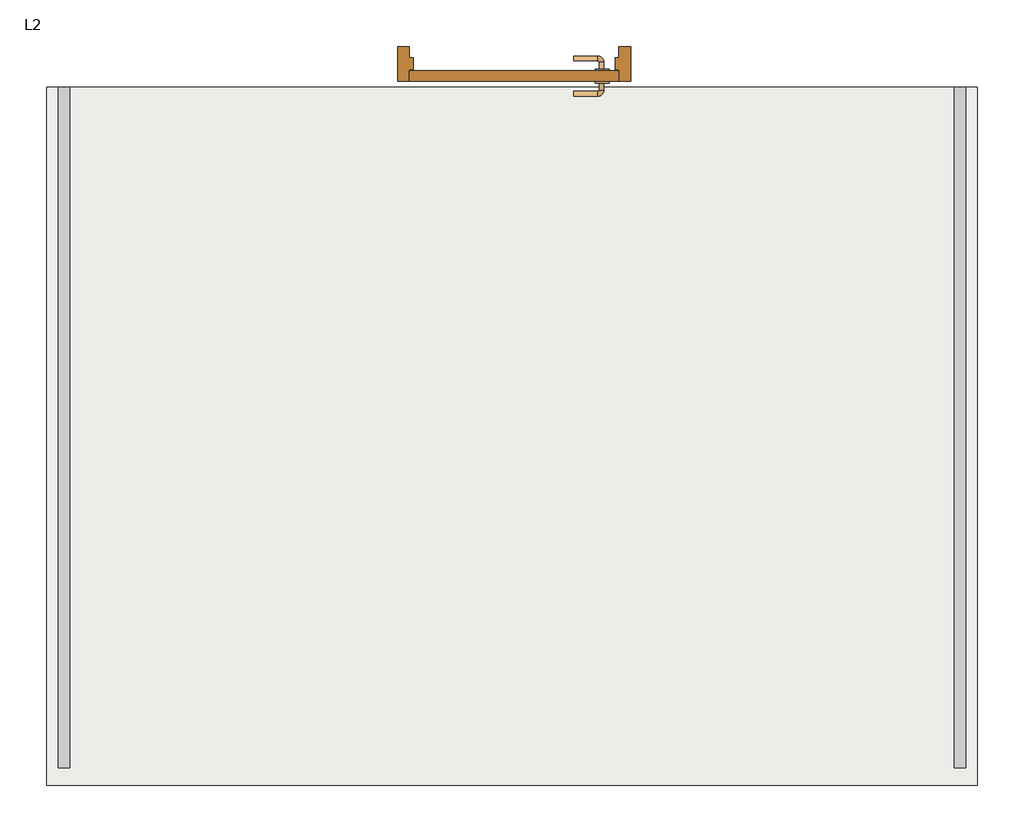
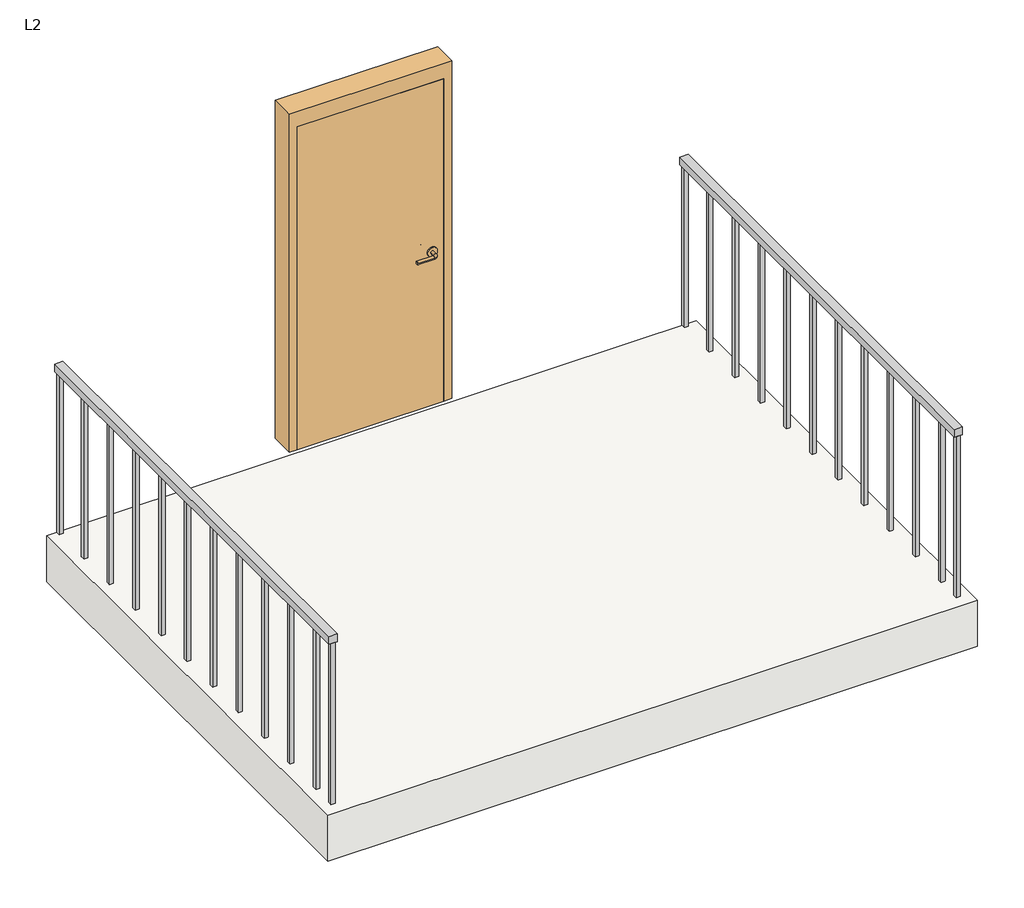
# One storey: 2 railings, 1 door, 1 slab.
"""IFC4 building model written with IfcOpenShell, lengths in millimetres."""

import ifcopenshell
import ifcopenshell.guid

model = None  # the IFC model being written
_history = None  # IfcOwnerHistory: only IFC2X3 demands one
_inside = {}  # id of a spatial element -> (the spatial element, [elements in it])
_under = {}  # id of a project, library or spatial element -> (it, [spatial elements below it])
_declared = {}  # id of a project -> (the project, [libraries it declares])
_typed = {}  # id of a type object -> (the type object, [elements of that type])
_made_of = {}  # id of a material, layer set ... -> (it, [elements and type objects made of it])


def new_model(schema):
    """Start an empty IFC model of exactly this schema.

    Asked for "IFC4X3", IfcOpenShell would pick the latest addendum, in which some entities
    have other attributes; the version numbers below select the first issue.
    IFC2X3 requires an IfcOwnerHistory on every rooted entity: one is made here for all.
    """
    global model, _history
    if schema == "IFC4X3":
        model = ifcopenshell.file(schema_version=(4, 3, 0, 0))
    else:
        model = ifcopenshell.file(schema=schema)
    _inside.clear()
    _under.clear()
    _declared.clear()
    _typed.clear()
    _made_of.clear()
    _history = None
    if model.schema == "IFC2X3":
        org = make("IfcOrganization", Name="unknown")
        user = make(
            "IfcPersonAndOrganization",
            ThePerson=make("IfcPerson", FamilyName="unknown"),
            TheOrganization=org,
        )
        app = make(
            "IfcApplication",
            ApplicationDeveloper=org,
            Version="unknown",
            ApplicationFullName="unknown",
            ApplicationIdentifier="unknown",
        )
        _history = make(
            "IfcOwnerHistory",
            OwningUser=user,
            OwningApplication=app,
            ChangeAction="ADDED",
            CreationDate=0,
        )
    return model


def make(cls, **values):
    """One entity of the class cls with the attributes given. An attribute that is None is left unset."""
    return model.create_entity(
        cls, **{name: value for name, value in values.items() if value is not None}
    )


def rooted(cls, **values):
    """An entity with a GlobalId (a new one), such as an element, a storey or a relation."""
    return make(cls, GlobalId=ifcopenshell.guid.new(), OwnerHistory=_history, **values)


def si_unit(unit_type, name, prefix=None):
    """IfcSIUnit, for example si_unit("LENGTHUNIT", "METRE", prefix="MILLI")."""
    return make("IfcSIUnit", UnitType=unit_type, Prefix=prefix, Name=name)


def assignment(units):
    """IfcUnitAssignment: the units of a project."""
    return None if units is None else make("IfcUnitAssignment", Units=units)


def point(xyz):
    """IfcCartesianPoint."""
    return None if xyz is None else make("IfcCartesianPoint", Coordinates=xyz)


def direction(xyz):
    """IfcDirection."""
    return None if xyz is None else make("IfcDirection", DirectionRatios=xyz)


def frame(location, z_axis=None, x_axis=None):
    """IfcAxis2Placement3D, a coordinate frame: its origin and axes. An axis left out is left unset."""
    return make(
        "IfcAxis2Placement3D",
        Location=point(location),
        Axis=direction(z_axis),
        RefDirection=direction(x_axis),
    )


def frame_2d(location, x_axis=None):
    """IfcAxis2Placement2D, a coordinate frame in the plane: its origin and x axis."""
    return make(
        "IfcAxis2Placement2D", Location=point(location), RefDirection=direction(x_axis)
    )


def origin():
    """The frame at (0, 0, 0) with its axes left unset."""
    return frame((0.0, 0.0, 0.0))


def origin_with_axes():
    """The frame at (0, 0, 0) with the z axis (0, 0, 1) and the x axis (1, 0, 0) written out."""
    return frame((0.0, 0.0, 0.0), z_axis=(0.0, 0.0, 1.0), x_axis=(1.0, 0.0, 0.0))


def place(relative_to, where):
    """IfcLocalPlacement: puts the frame where relative to a parent placement (None: the world)."""
    return make(
        "IfcLocalPlacement", PlacementRelTo=relative_to, RelativePlacement=where
    )


def context(
    kind, dimensions, precision=None, world=None, true_north=None, identifier=None
):
    """IfcGeometricRepresentationContext, for example the 3D "Model" context."""
    return make(
        "IfcGeometricRepresentationContext",
        ContextIdentifier=identifier,
        ContextType=kind,
        CoordinateSpaceDimension=dimensions,
        Precision=precision,
        WorldCoordinateSystem=world,
        TrueNorth=true_north,
    )


def project(units=None, contexts=None):
    """IfcProject with its units and contexts."""
    return rooted(
        "IfcProject",
        Name="project",
        RepresentationContexts=contexts,
        UnitsInContext=assignment(units),
    )


def spatial(cls, under=None, at=None, **own):
    """A site, building, storey or space (cls), placed at a placement, below another one or the project."""
    s = rooted(cls, ObjectPlacement=at, **own)
    if under is not None:
        _under.setdefault(under.id(), (under, []))[1].append(s)
    return s


def polyline(points):
    """IfcPolyline through the points."""
    return make("IfcPolyline", Points=[point(p) for p in points])


def circle_curve(where, radius):
    """IfcCircle in the frame where."""
    return make("IfcCircle", Position=where, Radius=radius)


def ellipse_curve(where, semi_axis1, semi_axis2):
    """IfcEllipse in the frame where."""
    return make(
        "IfcEllipse", Position=where, SemiAxis1=semi_axis1, SemiAxis2=semi_axis2
    )


def trimmed(basis, trim1, trim2, sense, master):
    """IfcTrimmedCurve: the piece of a basis curve between two trims."""
    return make(
        "IfcTrimmedCurve",
        BasisCurve=basis,
        Trim1=trim1,
        Trim2=trim2,
        SenseAgreement=sense,
        MasterRepresentation=master,
    )


def segment(curve, same_sense, transition):
    """IfcCompositeCurveSegment."""
    return make(
        "IfcCompositeCurveSegment",
        Transition=transition,
        SameSense=same_sense,
        ParentCurve=curve,
    )


def composite_curve(segments, self_intersect=None):
    """IfcCompositeCurve: segments joined end to end."""
    return make("IfcCompositeCurve", Segments=segments, SelfIntersect=self_intersect)


def outline(outer, holes=None, kind="AREA"):
    """IfcArbitraryClosedProfileDef: a profile drawn as a closed curve; with holes, ...WithVoids."""
    if holes is None:
        return make("IfcArbitraryClosedProfileDef", ProfileType=kind, OuterCurve=outer)
    return make(
        "IfcArbitraryProfileDefWithVoids",
        ProfileType=kind,
        OuterCurve=outer,
        InnerCurves=holes,
    )


def extrude(swept, where, along, depth):
    """IfcExtrudedAreaSolid: the profile swept, set in the frame where, extruded along a direction by depth."""
    return make(
        "IfcExtrudedAreaSolid",
        SweptArea=swept,
        Position=where,
        ExtrudedDirection=direction(along),
        Depth=depth,
    )


def faces_of(points, faces, orient=None, outer=None):
    """IfcFace entities. A face is a list of loops; a loop is a list of indices into points, from 0.

    orient and outer hold one flag for each loop. By default every Orientation is true, the
    first loop of a face is its IfcFaceOuterBound and the others are IfcFaceBound.
    """
    made = []
    for i, loops in enumerate(faces):
        bounds = []
        for j, loop in enumerate(loops):
            is_outer = j == 0 if outer is None else outer[i][j]
            bounds.append(
                make(
                    "IfcFaceOuterBound" if is_outer else "IfcFaceBound",
                    Bound=make("IfcPolyLoop", Polygon=[points[k] for k in loop]),
                    Orientation=True if orient is None else orient[i][j],
                )
            )
        made.append(make("IfcFace", Bounds=bounds))
    return made


def faceted_brep(points, faces, orient=None, outer=None, voids=None):
    """IfcFacetedBrep: a solid bounded by flat faces; with voids (closed shells), ...WithVoids."""
    shared = [point(p) for p in points]
    hull = make("IfcClosedShell", CfsFaces=faces_of(shared, faces, orient, outer))
    if voids is None:
        return make("IfcFacetedBrep", Outer=hull)
    return make(
        "IfcFacetedBrepWithVoids",
        Outer=hull,
        Voids=[
            make(cls, CfsFaces=faces_of(shared, fs, o, b)) for cls, fs, o, b in voids
        ],
    )


def shape(context_of_items, identifier, shape_type, items):
    """IfcShapeRepresentation: the items that make up one representation, for example the "Body"."""
    return make(
        "IfcShapeRepresentation",
        ContextOfItems=context_of_items,
        RepresentationIdentifier=identifier,
        RepresentationType=shape_type,
        Items=items,
    )


def source(mapping_origin, context_of_items, identifier, shape_type, items):
    """IfcRepresentationMap: a shape defined once, which mapped items show again and again."""
    return make(
        "IfcRepresentationMap",
        MappingOrigin=mapping_origin,
        MappedRepresentation=shape(context_of_items, identifier, shape_type, items),
    )


def transform(
    local_origin,
    x_axis=None,
    y_axis=None,
    z_axis=None,
    scale=None,
    scale2=None,
    scale3=None,
    uniform=True,
):
    """IfcCartesianTransformationOperator3D, or its non-uniform kind. x_axis, y_axis, z_axis: its Axis1, 2, 3."""
    if uniform:
        return make(
            "IfcCartesianTransformationOperator3D",
            Axis1=direction(x_axis),
            Axis2=direction(y_axis),
            LocalOrigin=point(local_origin),
            Scale=scale,
            Axis3=direction(z_axis),
        )
    return make(
        "IfcCartesianTransformationOperator3DnonUniform",
        Axis1=direction(x_axis),
        Axis2=direction(y_axis),
        LocalOrigin=point(local_origin),
        Scale=scale,
        Axis3=direction(z_axis),
        Scale2=scale2,
        Scale3=scale3,
    )


def mapped(mapping_source, mapping_target):
    """IfcMappedItem: shows the shape of a source again, moved by a transform."""
    return make(
        "IfcMappedItem", MappingSource=mapping_source, MappingTarget=mapping_target
    )


def made_of(thing, what):
    """Note that an element or type object is made of a material, layer set ...; save() writes the relation."""
    if what is not None:
        _made_of.setdefault(what.id(), (what, []))[1].append(thing)
    return thing


def element(
    cls,
    number,
    at=None,
    inside=None,
    cuts=None,
    type_object=None,
    material=None,
    context=None,
    identifier="Body",
    shape_type=None,
    held_by="IfcProductDefinitionShape",
    body=None,
    shapes=None,
    **own,
):
    """One element of the class cls, such as IfcWall. Its Tag is "e" and its number.

    at: its placement. inside: the storey or other place that contains it. cuts: it is an
    opening in that element (IfcRelVoidsElement). A single representation is given by context,
    identifier, shape_type and body (its items); several are given by shapes. held_by: the class
    of the entity that holds the representations. save() writes the other relations.
    """
    e = rooted(cls, Tag="e%d" % number, ObjectPlacement=at, **own)
    if body is not None:
        shapes = [shape(context, identifier, shape_type, body)]
    if shapes is not None:
        e.Representation = make(held_by, Representations=shapes)
    if inside is not None:
        _inside.setdefault(inside.id(), (inside, []))[1].append(e)
    if cuts is not None:
        rooted(
            "IfcRelVoidsElement", RelatingBuildingElement=cuts, RelatedOpeningElement=e
        )
    if type_object is not None:
        _typed.setdefault(type_object.id(), (type_object, []))[1].append(e)
    return made_of(e, material)


def aggregate(whole, parts):
    """IfcRelAggregates: a whole, such as a stair, and the parts it consists of."""
    return rooted("IfcRelAggregates", RelatingObject=whole, RelatedObjects=parts)


def save(model, path):
    """Write the relations noted so far, then the file.

    IfcRelAggregates (storeys below a building ...), IfcRelContainedInSpatialStructure (elements
    in a storey), IfcRelDefinesByType, IfcRelAssociatesMaterial and IfcRelDeclares: one each for
    every whole, place, type object, material and project.
    """
    for whole, parts in _under.values():
        aggregate(whole, parts)
    for where, things in _inside.values():
        rooted(
            "IfcRelContainedInSpatialStructure",
            RelatedElements=things,
            RelatingStructure=where,
        )
    for kind, things in _typed.values():
        rooted("IfcRelDefinesByType", RelatedObjects=things, RelatingType=kind)
    for what, things in _made_of.values():
        rooted("IfcRelAssociatesMaterial", RelatedObjects=things, RelatingMaterial=what)
    for by, libraries in _declared.values():
        rooted("IfcRelDeclares", RelatingContext=by, RelatedDefinitions=libraries)
    model.write(path)


def plane_surface(at):
    """IfcPlane: the flat surface through the origin of the frame at, square to its z axis."""
    return make("IfcPlane", Position=at)


def cylinder_surface(at, radius):
    """IfcCylindricalSurface: all points at the distance radius from the z axis of the frame at."""
    return make("IfcCylindricalSurface", Position=at, Radius=radius)


def revolved_surface(curve, axis_point, axis_direction):
    """IfcSurfaceOfRevolution: the curve turned about the line through axis_point along axis_direction."""
    return make(
        "IfcSurfaceOfRevolution",
        SweptCurve=make("IfcArbitraryOpenProfileDef", ProfileType="CURVE", Curve=curve),
        AxisPosition=make("IfcAxis1Placement", Location=point(axis_point), Axis=direction(axis_direction)),
    )


def advanced_brep(points, edges, surfaces, faces):
    """IfcAdvancedBrep: a solid bounded by faces that lie on surfaces and meet in shared edges.

    An edge is (start, end): straight between two places in points (the first is 0);
    or (start, end, curve); or (start, end, curve, False) where it runs against its curve.
    A face is (place in surfaces, loops), or (place, loops, False) where it looks against
    its surface's normal. A loop lists edges by number (the first is 1), with a minus sign
    where the edge is run from its end to its start. The first loop is the outer one.
    """
    corners = [point(p) for p in points]
    vertices = [make("IfcVertexPoint", VertexGeometry=c) for c in corners]
    made = []
    for start, end, *more in edges:
        made.append(
            make(
                "IfcEdgeCurve",
                EdgeStart=vertices[start],
                EdgeEnd=vertices[end],
                EdgeGeometry=more[0] if more else make("IfcPolyline", Points=[corners[start], corners[end]]),
                SameSense=more[1] if len(more) > 1 else True,
            )
        )
    hull = []
    for where, loops, *sense in faces:
        bounds = []
        for j, loop in enumerate(loops):
            ring = [make("IfcOrientedEdge", EdgeElement=made[abs(k) - 1], Orientation=k > 0) for k in loop]
            bounds.append(
                make(
                    "IfcFaceOuterBound" if j == 0 else "IfcFaceBound",
                    Bound=make("IfcEdgeLoop", EdgeList=ring),
                    Orientation=True,
                )
            )
        hull.append(make("IfcAdvancedFace", Bounds=bounds, FaceSurface=surfaces[where], SameSense=sense[0] if sense else True))
    return make("IfcAdvancedBrep", Outer=make("IfcClosedShell", CfsFaces=hull))


def m_door_passage_single_flush_900_x_2100mm_f70d95c9(model_context):
    return source(origin(), model_context, "Body", "SolidModel", [
        advanced_brep(
        [(-384.990625, 3.35, 1000.0), (-364.990625, 3.35, 1000.0), (-364.990625, -26.65, 1000.0), (-384.990625, -26.65, 1000.0), (-359.990625, -31.65, 1000.0), (-359.990625, -51.65, 1000.0), (-254.990625, -51.65, 1000.0), (-254.990625, -31.65, 1000.0)],
        [
            (0, 1, circle_curve(frame((-374.990625, 3.35, 1000.0), z_axis=(0.0, 1.0, 0.0), x_axis=(1.0, 0.0, 0.0)), 10.0)),
            (1, 0, circle_curve(frame((-374.990625, 3.35, 1000.0), z_axis=(0.0, 1.0, 0.0), x_axis=(1.0, 0.0, 0.0)), 10.0)),
            (1, 2),
            (2, 3, circle_curve(frame((-374.990625, -26.65, 1000.0), z_axis=(0.0, 1.0, 0.0), x_axis=(1.0, 0.0, 0.0)), 10.0)),
            (3, 0),
            (3, 2, circle_curve(frame((-374.990625, -26.65, 1000.0), z_axis=(0.0, 1.0, 0.0), x_axis=(1.0, 0.0, 0.0)), 10.0)),
            (4, 5, circle_curve(frame((-359.990625, -41.65, 1000.0), z_axis=(-1.0, 0.0, 0.0), x_axis=(0.0, 1.0, 0.0)), 10.0)),
            (5, 3, circle_curve(frame((-359.990625, -26.65, 1000.0), z_axis=(0.0, 0.0, -1.0), x_axis=(-1.0, 0.0, 0.0)), 25.0)),
            (2, 4, circle_curve(frame((-359.990625, -26.65, 1000.0), z_axis=(0.0, 0.0, 1.0), x_axis=(-1.0, 0.0, 0.0)), 5.0)),
            (5, 4, circle_curve(frame((-359.990625, -41.65, 1000.0), z_axis=(-1.0, 0.0, 0.0), x_axis=(0.0, 1.0, 0.0)), 10.0)),
            (6, 7, circle_curve(frame((-254.990625, -41.65, 1000.0), z_axis=(1.0, 0.0, 0.0), x_axis=(0.0, 1.0, 0.0)), 10.0)),
            (7, 6, circle_curve(frame((-254.990625, -41.65, 1000.0), z_axis=(1.0, 0.0, 0.0), x_axis=(0.0, 1.0, 0.0)), 10.0)),
            (4, 7),
            (6, 5),
        ],
        [
            plane_surface(frame((-374.990625, 3.35, 1000.0), z_axis=(0.0, 1.0, 0.0), x_axis=(0.0, 0.0, 1.0))),
            cylinder_surface(frame((-374.990625, 3.35, 1000.0), z_axis=(0.0, 1.0, 0.0), x_axis=(1.0, 0.0, 0.0)), 10.0),
            revolved_surface(trimmed(ellipse_curve(frame((-374.990625, -26.65, 1000.0), z_axis=(0.0, -1.0, 0.0), x_axis=(1.0, 0.0, 0.0)), 10.0, 10.0), [point((-384.990625, -26.65, 1000.0))], [point((-364.990625, -26.65, 1000.0))], True, "CARTESIAN"), (-359.990625, -26.65, 1000.0), (0.0, 0.0, -1.0)),
            revolved_surface(trimmed(ellipse_curve(frame((-374.990625, -26.65, 1000.0), z_axis=(0.0, -1.0, 0.0), x_axis=(1.0, 0.0, 0.0)), 10.0, 10.0), [point((-364.990625, -26.65, 1000.0))], [point((-384.990625, -26.65, 1000.0))], True, "CARTESIAN"), (-359.990625, -26.65, 1000.0), (0.0, 0.0, -1.0)),
            plane_surface(frame((-254.990625, -41.65, 1000.0), z_axis=(1.0, 0.0, 0.0), x_axis=(0.0, 0.0, 1.0))),
            cylinder_surface(frame((-359.990625, -41.65, 1000.0), z_axis=(-1.0, 0.0, 0.0), x_axis=(0.0, 1.0, 0.0)), 10.0),
        ],
        [
            (0, [[1, 2]]),
            (1, [[3, 4, 5, -2]]),
            (1, [[-5, 6, -3, -1]]),
            (2, [[7, 8, -4, 9]]),
            (3, [[10, -9, -6, -8]]),
            (4, [[11, 12]]),
            (5, [[13, -11, 14, -7]]),
            (5, [[-14, -12, -13, -10]]),
        ],
    ),
        extrude(outline(composite_curve([segment(trimmed(circle_curve(frame_2d((1000.0, -377.490625)), 30.0), [point((1000.0, -407.490625))], [point((1000.0, -347.490625))], False, "CARTESIAN"), True, "CONTINUOUS"), segment(trimmed(circle_curve(frame_2d((1000.0, -377.490625)), 30.0), [point((1000.0, -347.490625))], [point((1000.0, -407.490625))], False, "CARTESIAN"), True, "CONTINUOUS")], self_intersect=False)), frame((0.0, 3.35, 0.0), z_axis=(0.0, 1.0, 0.0), x_axis=(0.0, 0.0, 1.0)), (0.0, 0.0, 1.0), 8.0),
        advanced_brep(
        [(-384.990625, 64.35, 1000.0), (-364.990625, 64.35, 1000.0), (-384.990625, 94.35, 1000.0), (-364.990625, 94.35, 1000.0), (-359.990625, 99.35, 1000.0), (-359.990625, 119.35, 1000.0), (-254.990625, 119.35, 1000.0), (-254.990625, 99.35, 1000.0)],
        [
            (0, 1, circle_curve(frame((-374.990625, 64.35, 1000.0), z_axis=(0.0, -1.0, 0.0), x_axis=(1.0, 0.0, 0.0)), 10.0)),
            (1, 0, circle_curve(frame((-374.990625, 64.35, 1000.0), z_axis=(0.0, -1.0, 0.0), x_axis=(1.0, 0.0, 0.0)), 10.0)),
            (0, 2),
            (2, 3, circle_curve(frame((-374.990625, 94.35, 1000.0), z_axis=(0.0, -1.0, 0.0), x_axis=(1.0, 0.0, 0.0)), 10.0)),
            (3, 1),
            (3, 2, circle_curve(frame((-374.990625, 94.35, 1000.0), z_axis=(0.0, -1.0, 0.0), x_axis=(1.0, 0.0, 0.0)), 10.0)),
            (4, 3, circle_curve(frame((-359.990625, 94.35, 1000.0), z_axis=(0.0, 0.0, 1.0), x_axis=(-1.0, 0.0, 0.0)), 5.0)),
            (2, 5, circle_curve(frame((-359.990625, 94.35, 1000.0), z_axis=(0.0, 0.0, -1.0), x_axis=(-1.0, 0.0, 0.0)), 25.0)),
            (5, 4, circle_curve(frame((-359.990625, 109.35, 1000.0), z_axis=(-1.0, 0.0, 0.0), x_axis=(0.0, -1.0, 0.0)), 10.0)),
            (4, 5, circle_curve(frame((-359.990625, 109.35, 1000.0), z_axis=(-1.0, 0.0, 0.0), x_axis=(0.0, -1.0, 0.0)), 10.0)),
            (6, 7, circle_curve(frame((-254.990625, 109.35, 1000.0), z_axis=(1.0, 0.0, 0.0), x_axis=(0.0, -1.0, 0.0)), 10.0)),
            (7, 6, circle_curve(frame((-254.990625, 109.35, 1000.0), z_axis=(1.0, 0.0, 0.0), x_axis=(0.0, -1.0, 0.0)), 10.0)),
            (5, 6),
            (7, 4),
        ],
        [
            plane_surface(frame((-374.990625, 64.35, 1000.0), z_axis=(0.0, -1.0, 0.0), x_axis=(0.0, 0.0, 1.0))),
            cylinder_surface(frame((-374.990625, 64.35, 1000.0), z_axis=(0.0, -1.0, 0.0), x_axis=(1.0, 0.0, 0.0)), 10.0),
            revolved_surface(trimmed(ellipse_curve(frame((-374.990625, 94.35, 1000.0), z_axis=(0.0, -1.0, 0.0), x_axis=(1.0, 0.0, 0.0)), 10.0, 10.0), [point((-384.990625, 94.35, 1000.0))], [point((-364.990625, 94.35, 1000.0))], True, "CARTESIAN"), (-359.990625, 94.35, 1000.0), (0.0, 0.0, -1.0)),
            revolved_surface(trimmed(ellipse_curve(frame((-374.990625, 94.35, 1000.0), z_axis=(0.0, -1.0, 0.0), x_axis=(1.0, 0.0, 0.0)), 10.0, 10.0), [point((-364.990625, 94.35, 1000.0))], [point((-384.990625, 94.35, 1000.0))], True, "CARTESIAN"), (-359.990625, 94.35, 1000.0), (0.0, 0.0, -1.0)),
            plane_surface(frame((-254.990625, 109.35, 1000.0), z_axis=(1.0, 0.0, 0.0), x_axis=(0.0, 0.0, 1.0))),
            cylinder_surface(frame((-359.990625, 109.35, 1000.0), z_axis=(-1.0, 0.0, 0.0), x_axis=(0.0, -1.0, 0.0)), 10.0),
        ],
        [
            (0, [[1, 2]]),
            (1, [[-1, 3, 4, 5]]),
            (1, [[-2, -5, 6, -3]]),
            (2, [[7, -4, 8, 9]]),
            (3, [[-8, -6, -7, 10]]),
            (4, [[11, 12]]),
            (5, [[-9, 13, -12, 14]]),
            (5, [[-10, -14, -11, -13]]),
        ],
    ),
        extrude(outline(composite_curve([segment(trimmed(circle_curve(frame_2d((1000.0, -377.490625)), 30.0), [point((1000.0, -407.490625))], [point((1000.0, -347.490625))], False, "CARTESIAN"), True, "CONTINUOUS"), segment(trimmed(circle_curve(frame_2d((1000.0, -377.490625)), 30.0), [point((1000.0, -347.490625))], [point((1000.0, -407.490625))], False, "CARTESIAN"), True, "CONTINUOUS")], self_intersect=False)), frame((0.0, 56.35, 0.0), z_axis=(0.0, 1.0, 0.0), x_axis=(0.0, 0.0, 1.0)), (0.0, 0.0, 1.0), 8.0),
        extrude(outline(polyline([(450.0, 11.35), (-450.0, 11.35), (-450.0, 56.35), (450.0, 56.35), (450.0, 11.35)])), origin_with_axes(), (0.0, 0.0, 1.0), 2100.0),
        faceted_brep([(450.0, 6.5875, 0.0), (450.0, 56.35, 0.0), (500.0, 56.35, 0.0), (500.0, -93.65, 0.0), (450.0, -93.65, 0.0), (450.0, -44.4375, 0.0), (434.125, -44.4375, 0.0), (434.125, 6.5875, 0.0), (450.0, 6.5875, 2100.0), (450.0, 56.35, 2100.0), (-450.0, 56.35, 2100.0), (-450.0, 56.35, 0.0), (-500.0, 56.35, 0.0), (-500.0, 56.35, 2200.0), (500.0, 56.35, 2200.0), (500.0, -93.65, 2200.0), (-500.0, -93.65, 2200.0), (-500.0, -93.65, 0.0), (-450.0, -93.65, 0.0), (-450.0, -93.65, 2100.0), (450.0, -93.65, 2100.0), (450.0, -44.4375, 2100.0), (-450.0, -44.4375, 2100.0), (-450.0, -44.4375, 0.0), (-434.125, -44.4375, 0.0), (-434.125, -44.4375, 2084.125), (434.125, -44.4375, 2084.125), (434.125, 6.5875, 2084.125), (-434.125, 6.5875, 2084.125), (-434.125, 6.5875, 0.0), (-450.0, 6.5875, 0.0), (-450.0, 6.5875, 2100.0)], [[[0, 1, 2, 3, 4, 5, 6, 7]], [[1, 0, 8, 9]], [[2, 1, 9, 10, 11, 12, 13, 14]], [[3, 2, 14, 15]], [[4, 3, 15, 16, 17, 18, 19, 20]], [[5, 4, 20, 21]], [[6, 5, 21, 22, 23, 24, 25, 26]], [[7, 6, 26, 27]], [[0, 7, 27, 28, 29, 30, 31, 8]], [[9, 8, 31, 10]], [[20, 19, 22, 21]], [[26, 25, 28, 27]], [[12, 11, 30, 29, 24, 23, 18, 17]], [[11, 10, 31, 30]], [[13, 12, 17, 16]], [[19, 18, 23, 22]], [[25, 24, 29, 28]], [[15, 14, 13, 16]]]),
    ])


model = new_model("IFC4")

# Units and contexts
model_context = context("Model", 3, world=origin())
ifc_project = project(units=[si_unit("LENGTHUNIT", "METRE", prefix="MILLI")], contexts=[model_context])

# Site, building, storey
site = spatial("IfcSite", under=ifc_project)
building = spatial("IfcBuilding", under=site)
storey = spatial("IfcBuildingStorey", under=building, Name="L2", Elevation=1200.0)

# Door
placement = place(None, origin())
m_door_passage_single_flush_900_x_2100mm_shape = m_door_passage_single_flush_900_x_2100mm_f70d95c9(model_context)
element("IfcDoor", 1, ObjectType="M_Door-Passage-Single-Flush : 900 x 2100mm", at=placement, inside=storey, context=model_context, shape_type="MappedRepresentation", body=[
    mapped(m_door_passage_single_flush_900_x_2100mm_shape, transform((752.7568, 2222.9207088, 1200.0), x_axis=(-1.0, 0.0, 0.0), y_axis=(0.0, -1.0, 0.0), z_axis=(0.0, 0.0, 1.0))),
])

# Railings
element("IfcRailing", 2, ObjectType="1100mm", at=placement, inside=storey, context=model_context, shape_type="SweptSolid", body=[
    extrude(outline(polyline([(-1206.7682, 2141.5707088), (-1156.7682, 2141.5707088), (-1156.7682, -783.4292912), (-1206.7682, -783.4292912), (-1206.7682, 2141.5707088)])), frame((0.0, 0.0, 2250.0), z_axis=(0.0, 0.0, 1.0), x_axis=(1.0, 0.0, 0.0)), (0.0, 0.0, 1.0), 50.0),
    extrude(outline(polyline([(-1194.2682, -595.9292912), (-1169.2682, -595.9292912), (-1169.2682, -620.9292912), (-1194.2682, -620.9292912), (-1194.2682, -595.9292912)])), frame((0.0, 0.0, 1200.0), z_axis=(0.0, 0.0, 1.0), x_axis=(1.0, 0.0, 0.0)), (0.0, 0.0, 1.0), 1050.0),
    extrude(outline(polyline([(-1194.2682, -320.9292912), (-1169.2682, -320.9292912), (-1169.2682, -345.9292912), (-1194.2682, -345.9292912), (-1194.2682, -320.9292912)])), frame((0.0, 0.0, 1200.0), z_axis=(0.0, 0.0, 1.0), x_axis=(1.0, 0.0, 0.0)), (0.0, 0.0, 1.0), 1050.0),
    extrude(outline(polyline([(-1194.2682, -45.9292912), (-1169.2682, -45.9292912), (-1169.2682, -70.9292912), (-1194.2682, -70.9292912), (-1194.2682, -45.9292912)])), frame((0.0, 0.0, 1200.0), z_axis=(0.0, 0.0, 1.0), x_axis=(1.0, 0.0, 0.0)), (0.0, 0.0, 1.0), 1050.0),
    extrude(outline(polyline([(-1194.2682, 229.0707088), (-1169.2682, 229.0707088), (-1169.2682, 204.0707088), (-1194.2682, 204.0707088), (-1194.2682, 229.0707088)])), frame((0.0, 0.0, 1200.0), z_axis=(0.0, 0.0, 1.0), x_axis=(1.0, 0.0, 0.0)), (0.0, 0.0, 1.0), 1050.0),
    extrude(outline(polyline([(-1194.2682, 504.0707088), (-1169.2682, 504.0707088), (-1169.2682, 479.0707088), (-1194.2682, 479.0707088), (-1194.2682, 504.0707088)])), frame((0.0, 0.0, 1200.0), z_axis=(0.0, 0.0, 1.0), x_axis=(1.0, 0.0, 0.0)), (0.0, 0.0, 1.0), 1050.0),
    extrude(outline(polyline([(-1194.2682, 779.0707088), (-1169.2682, 779.0707088), (-1169.2682, 754.0707088), (-1194.2682, 754.0707088), (-1194.2682, 779.0707088)])), frame((0.0, 0.0, 1200.0), z_axis=(0.0, 0.0, 1.0), x_axis=(1.0, 0.0, 0.0)), (0.0, 0.0, 1.0), 1050.0),
    extrude(outline(polyline([(-1194.2682, 1054.0707088), (-1169.2682, 1054.0707088), (-1169.2682, 1029.0707088), (-1194.2682, 1029.0707088), (-1194.2682, 1054.0707088)])), frame((0.0, 0.0, 1200.0), z_axis=(0.0, 0.0, 1.0), x_axis=(1.0, 0.0, 0.0)), (0.0, 0.0, 1.0), 1050.0),
    extrude(outline(polyline([(-1194.2682, 1329.0707088), (-1169.2682, 1329.0707088), (-1169.2682, 1304.0707088), (-1194.2682, 1304.0707088), (-1194.2682, 1329.0707088)])), frame((0.0, 0.0, 1200.0), z_axis=(0.0, 0.0, 1.0), x_axis=(1.0, 0.0, 0.0)), (0.0, 0.0, 1.0), 1050.0),
    extrude(outline(polyline([(-1194.2682, 1604.0707088), (-1169.2682, 1604.0707088), (-1169.2682, 1579.0707088), (-1194.2682, 1579.0707088), (-1194.2682, 1604.0707088)])), frame((0.0, 0.0, 1200.0), z_axis=(0.0, 0.0, 1.0), x_axis=(1.0, 0.0, 0.0)), (0.0, 0.0, 1.0), 1050.0),
    extrude(outline(polyline([(-1194.2682, 1879.0707088), (-1169.2682, 1879.0707088), (-1169.2682, 1854.0707088), (-1194.2682, 1854.0707088), (-1194.2682, 1879.0707088)])), frame((0.0, 0.0, 1200.0), z_axis=(0.0, 0.0, 1.0), x_axis=(1.0, 0.0, 0.0)), (0.0, 0.0, 1.0), 1050.0),
    extrude(outline(polyline([(-1194.2682, -758.4292912), (-1169.2682, -758.4292912), (-1169.2682, -783.4292912), (-1194.2682, -783.4292912), (-1194.2682, -758.4292912)])), frame((0.0, 0.0, 1200.0), z_axis=(0.0, 0.0, 1.0), x_axis=(1.0, 0.0, 0.0)), (0.0, 0.0, 1.0), 1050.0),
    extrude(outline(polyline([(-1194.2682, 2141.5707088), (-1169.2682, 2141.5707088), (-1169.2682, 2116.5707088), (-1194.2682, 2116.5707088), (-1194.2682, 2141.5707088)])), frame((0.0, 0.0, 1200.0), z_axis=(0.0, 0.0, 1.0), x_axis=(1.0, 0.0, 0.0)), (0.0, 0.0, 1.0), 1050.0),
])
element("IfcRailing", 3, ObjectType="1100mm", at=placement, inside=storey, context=model_context, shape_type="SweptSolid", body=[
    extrude(outline(polyline([(2643.2318, 2141.5707088), (2693.2318, 2141.5707088), (2693.2318, -783.4292912), (2643.2318, -783.4292912), (2643.2318, 2141.5707088)])), frame((0.0, 0.0, 2250.0), z_axis=(0.0, 0.0, 1.0), x_axis=(1.0, 0.0, 0.0)), (0.0, 0.0, 1.0), 50.0),
    extrude(outline(polyline([(2655.7318, -595.9292912), (2680.7318, -595.9292912), (2680.7318, -620.9292912), (2655.7318, -620.9292912), (2655.7318, -595.9292912)])), frame((0.0, 0.0, 1200.0), z_axis=(0.0, 0.0, 1.0), x_axis=(1.0, 0.0, 0.0)), (0.0, 0.0, 1.0), 1050.0),
    extrude(outline(polyline([(2655.7318, -320.9292912), (2680.7318, -320.9292912), (2680.7318, -345.9292912), (2655.7318, -345.9292912), (2655.7318, -320.9292912)])), frame((0.0, 0.0, 1200.0), z_axis=(0.0, 0.0, 1.0), x_axis=(1.0, 0.0, 0.0)), (0.0, 0.0, 1.0), 1050.0),
    extrude(outline(polyline([(2655.7318, -45.9292912), (2680.7318, -45.9292912), (2680.7318, -70.9292912), (2655.7318, -70.9292912), (2655.7318, -45.9292912)])), frame((0.0, 0.0, 1200.0), z_axis=(0.0, 0.0, 1.0), x_axis=(1.0, 0.0, 0.0)), (0.0, 0.0, 1.0), 1050.0),
    extrude(outline(polyline([(2655.7318, 229.0707088), (2680.7318, 229.0707088), (2680.7318, 204.0707088), (2655.7318, 204.0707088), (2655.7318, 229.0707088)])), frame((0.0, 0.0, 1200.0), z_axis=(0.0, 0.0, 1.0), x_axis=(1.0, 0.0, 0.0)), (0.0, 0.0, 1.0), 1050.0),
    extrude(outline(polyline([(2655.7318, 504.0707088), (2680.7318, 504.0707088), (2680.7318, 479.0707088), (2655.7318, 479.0707088), (2655.7318, 504.0707088)])), frame((0.0, 0.0, 1200.0), z_axis=(0.0, 0.0, 1.0), x_axis=(1.0, 0.0, 0.0)), (0.0, 0.0, 1.0), 1050.0),
    extrude(outline(polyline([(2655.7318, 779.0707088), (2680.7318, 779.0707088), (2680.7318, 754.0707088), (2655.7318, 754.0707088), (2655.7318, 779.0707088)])), frame((0.0, 0.0, 1200.0), z_axis=(0.0, 0.0, 1.0), x_axis=(1.0, 0.0, 0.0)), (0.0, 0.0, 1.0), 1050.0),
    extrude(outline(polyline([(2655.7318, 1054.0707088), (2680.7318, 1054.0707088), (2680.7318, 1029.0707088), (2655.7318, 1029.0707088), (2655.7318, 1054.0707088)])), frame((0.0, 0.0, 1200.0), z_axis=(0.0, 0.0, 1.0), x_axis=(1.0, 0.0, 0.0)), (0.0, 0.0, 1.0), 1050.0),
    extrude(outline(polyline([(2655.7318, 1329.0707088), (2680.7318, 1329.0707088), (2680.7318, 1304.0707088), (2655.7318, 1304.0707088), (2655.7318, 1329.0707088)])), frame((0.0, 0.0, 1200.0), z_axis=(0.0, 0.0, 1.0), x_axis=(1.0, 0.0, 0.0)), (0.0, 0.0, 1.0), 1050.0),
    extrude(outline(polyline([(2655.7318, 1604.0707088), (2680.7318, 1604.0707088), (2680.7318, 1579.0707088), (2655.7318, 1579.0707088), (2655.7318, 1604.0707088)])), frame((0.0, 0.0, 1200.0), z_axis=(0.0, 0.0, 1.0), x_axis=(1.0, 0.0, 0.0)), (0.0, 0.0, 1.0), 1050.0),
    extrude(outline(polyline([(2655.7318, 1879.0707088), (2680.7318, 1879.0707088), (2680.7318, 1854.0707088), (2655.7318, 1854.0707088), (2655.7318, 1879.0707088)])), frame((0.0, 0.0, 1200.0), z_axis=(0.0, 0.0, 1.0), x_axis=(1.0, 0.0, 0.0)), (0.0, 0.0, 1.0), 1050.0),
    extrude(outline(polyline([(2655.7318, -758.4292912), (2680.7318, -758.4292912), (2680.7318, -783.4292912), (2655.7318, -783.4292912), (2655.7318, -758.4292912)])), frame((0.0, 0.0, 1200.0), z_axis=(0.0, 0.0, 1.0), x_axis=(1.0, 0.0, 0.0)), (0.0, 0.0, 1.0), 1050.0),
    extrude(outline(polyline([(2655.7318, 2141.5707088), (2680.7318, 2141.5707088), (2680.7318, 2116.5707088), (2655.7318, 2116.5707088), (2655.7318, 2141.5707088)])), frame((0.0, 0.0, 1200.0), z_axis=(0.0, 0.0, 1.0), x_axis=(1.0, 0.0, 0.0)), (0.0, 0.0, 1.0), 1050.0),
])

# Slab
element("IfcSlab", 4, ObjectType="Generic 300mm", at=placement, inside=storey, context=model_context, shape_type="SweptSolid", body=[
    extrude(outline(polyline([(2743.2318, -858.4292912), (-1256.7682, -858.4292912), (-1256.7682, 2141.5707088), (2743.2318, 2141.5707088), (2743.2318, -858.4292912)])), frame((0.0, 0.0, 900.0), z_axis=(0.0, 0.0, 1.0), x_axis=(1.0, 0.0, 0.0)), (0.0, 0.0, 1.0), 300.0),
])

save(model, "model.ifc")

# Revit data of these elements
# Project information
#   Название организации = "Organization Name"
#   Описание организации = "Organization Description"
#   Наименование здания = "Building Name"
#   Дата утверждения проекта = "Issue Date"
#   Статус проекта = "Project Status"
#   Заказчик = "Client Name"
#   Адрес проекта = "Enter address here\nAddress Line 2"
#   Наименование проекта = "Project Name"
#   Номер проекта = "Project Number"
# Type "M_Door-Passage-Single-Flush : 900 x 2100mm"
#   Type Mark = "38"
#   Analytic Construction = "Wooden"
#   Thickness = 45 mm
#   Thermal Resistance (R) = 0.455703 (m²·K)/W
#   Swing Angle [instance default] = 90.00°
#   Strike Height = 1000 mm
#   Rough Width [instance default] = 1000 mm
#   Rough Height [instance default] = 2200 mm
#   MF Opening Height [instance default] = 100 mm
#   MF Opening Width [instance default] = 100 mm
#   Inset Calculate [instance default] = 105 mm
#   Masonry Inset [instance default] = 25 mm
#   Height = 2100 mm
#   Width = 900 mm
#   Heat Transfer Coefficient (U) = 2.19465 W/(m²·K)
#   Masonry Frame Depth = 150 mm
#   Masonry Frame [instance default] = yes
#   Function = 1
#   Dry Wall Frame [instance default] = no
#   Panel Material = Wood - Birch
#   Frame Material = Metal - Paint Finish - Grey
#   Door Handle Material = Aluminum
#   Visual Light Transmittance = 0
#   Solar Heat Gain Coefficient = 0
#   Wall Closure = (empty or 0)
# Type "1100mm"
#   built-in parameter 1008612 = 0.019685 (stored number, unit not read)
#   built-in parameter 1008611 = 0.019685 (stored number, unit not read)
#   built-in parameter 1008609 = 0.902231 (stored number, unit not read)
#   built-in parameter 1008604 = 0.19685 (stored number, unit not read)
#   built-in parameter 1008603 = 0.164042 (stored number, unit not read)
#   Railing Height = 1100 mm
#   built-in parameter 1008630 = 2
#   built-in parameter 1008610 = 2
#   built-in parameter 1008608 = 1
#   built-in parameter 1008618 = M_Baluster - Square : 25mm
# Type "Generic 300mm"
#   Description = "Generic Floor (Material By Category), 300mm thick"
#   Function = 0
#   Layers, outside or top first: 300 mm no material (function 1)
# Element 1 (IfcDoor, "M_Door-Passage-Single-Flush : 900 x 2100mm")
#   Swing Angle = 90.00°
#   Rough Width = 1000 mm
#   Rough Height = 2200 mm
#   Masonry Inset = 25 mm
#   MF Opening Width = 100 mm
#   MF Opening Height = 100 mm
#   Inset Calculate = 105 mm
#   Masonry Frame = yes
#   Dry Wall Frame = no
#   Phase Created = New Construction
#   Materials on its faces: "Aluminum", "Metal - Paint Finish - Grey", "Wood - Birch"
# Elements 2, 3 (IfcRailing, "1100mm")
#   Phase Created = New Construction
# Element 4 (IfcSlab, "Generic 300mm")
#   Height Offset From Level = 0 mm
#   Phase Created = New Construction
#   Materials on its faces: "Default Floor"
# Materials
#   "Wood - Birch": class "Wood", colour RGB 173 132 96, transparency 0, Cost = 0
#   "Metal - Paint Finish - Grey": class "Paint", colour RGB 178 178 178, transparency 0, Cost = 0
#   "Aluminum": class "Metal", colour RGB 244 245 246, transparency 0, Description = "Aluminum 6061", Cost = 0
#   "Default Floor": class "Miscellaneous", colour RGB 128 128 128, transparency 0, Cost = 0
